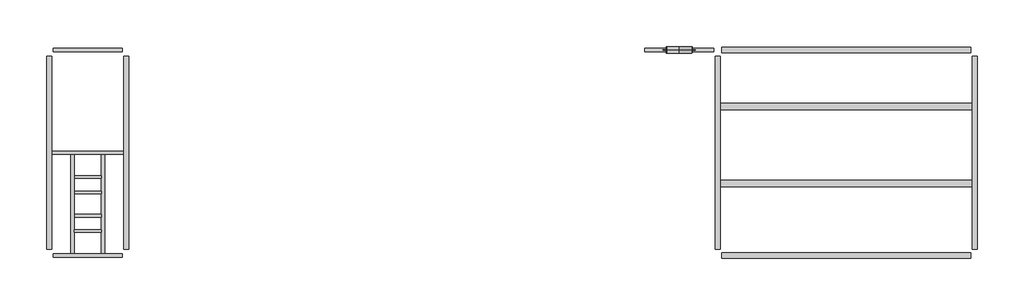
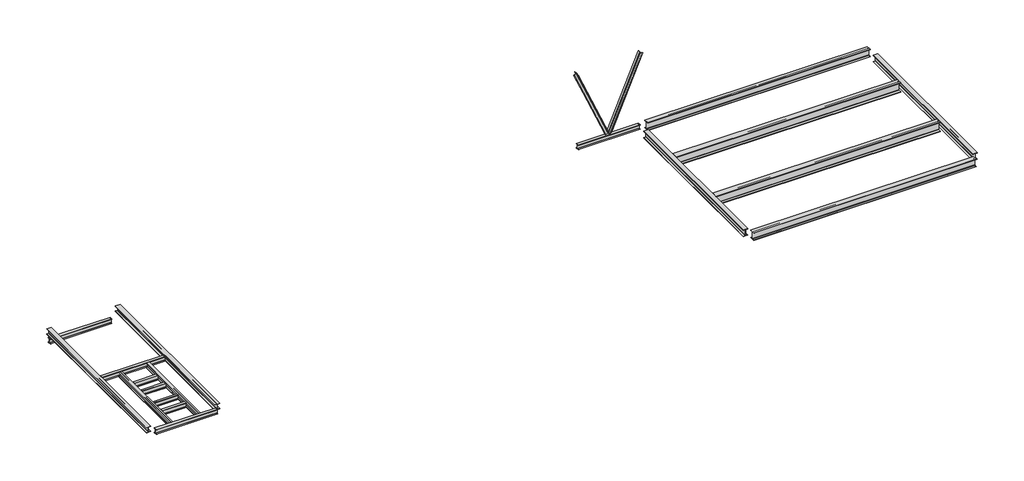
# One storey: 18 beams, 2 members.
"""IFC4 building model written with IfcOpenShell, lengths in millimetres."""

import ifcopenshell
import ifcopenshell.guid

model = None  # the IFC model being written
_history = None  # IfcOwnerHistory: only IFC2X3 demands one
_inside = {}  # id of a spatial element -> (the spatial element, [elements in it])
_under = {}  # id of a project, library or spatial element -> (it, [spatial elements below it])
_declared = {}  # id of a project -> (the project, [libraries it declares])
_typed = {}  # id of a type object -> (the type object, [elements of that type])
_made_of = {}  # id of a material, layer set ... -> (it, [elements and type objects made of it])


def new_model(schema):
    """Start an empty IFC model of exactly this schema.

    Asked for "IFC4X3", IfcOpenShell would pick the latest addendum, in which some entities
    have other attributes; the version numbers below select the first issue.
    IFC2X3 requires an IfcOwnerHistory on every rooted entity: one is made here for all.
    """
    global model, _history
    if schema == "IFC4X3":
        model = ifcopenshell.file(schema_version=(4, 3, 0, 0))
    else:
        model = ifcopenshell.file(schema=schema)
    _inside.clear()
    _under.clear()
    _declared.clear()
    _typed.clear()
    _made_of.clear()
    _history = None
    if model.schema == "IFC2X3":
        org = make("IfcOrganization", Name="unknown")
        user = make(
            "IfcPersonAndOrganization",
            ThePerson=make("IfcPerson", FamilyName="unknown"),
            TheOrganization=org,
        )
        app = make(
            "IfcApplication",
            ApplicationDeveloper=org,
            Version="unknown",
            ApplicationFullName="unknown",
            ApplicationIdentifier="unknown",
        )
        _history = make(
            "IfcOwnerHistory",
            OwningUser=user,
            OwningApplication=app,
            ChangeAction="ADDED",
            CreationDate=0,
        )
    return model


def make(cls, **values):
    """One entity of the class cls with the attributes given. An attribute that is None is left unset."""
    return model.create_entity(
        cls, **{name: value for name, value in values.items() if value is not None}
    )


def rooted(cls, **values):
    """An entity with a GlobalId (a new one), such as an element, a storey or a relation."""
    return make(cls, GlobalId=ifcopenshell.guid.new(), OwnerHistory=_history, **values)


def si_unit(unit_type, name, prefix=None):
    """IfcSIUnit, for example si_unit("LENGTHUNIT", "METRE", prefix="MILLI")."""
    return make("IfcSIUnit", UnitType=unit_type, Prefix=prefix, Name=name)


def assignment(units):
    """IfcUnitAssignment: the units of a project."""
    return None if units is None else make("IfcUnitAssignment", Units=units)


def point(xyz):
    """IfcCartesianPoint."""
    return None if xyz is None else make("IfcCartesianPoint", Coordinates=xyz)


def direction(xyz):
    """IfcDirection."""
    return None if xyz is None else make("IfcDirection", DirectionRatios=xyz)


def frame(location, z_axis=None, x_axis=None):
    """IfcAxis2Placement3D, a coordinate frame: its origin and axes. An axis left out is left unset."""
    return make(
        "IfcAxis2Placement3D",
        Location=point(location),
        Axis=direction(z_axis),
        RefDirection=direction(x_axis),
    )


def frame_2d(location, x_axis=None):
    """IfcAxis2Placement2D, a coordinate frame in the plane: its origin and x axis."""
    return make(
        "IfcAxis2Placement2D", Location=point(location), RefDirection=direction(x_axis)
    )


def origin():
    """The frame at (0, 0, 0) with its axes left unset."""
    return frame((0.0, 0.0, 0.0))


def place(relative_to, where):
    """IfcLocalPlacement: puts the frame where relative to a parent placement (None: the world)."""
    return make(
        "IfcLocalPlacement", PlacementRelTo=relative_to, RelativePlacement=where
    )


def context(
    kind, dimensions, precision=None, world=None, true_north=None, identifier=None
):
    """IfcGeometricRepresentationContext, for example the 3D "Model" context."""
    return make(
        "IfcGeometricRepresentationContext",
        ContextIdentifier=identifier,
        ContextType=kind,
        CoordinateSpaceDimension=dimensions,
        Precision=precision,
        WorldCoordinateSystem=world,
        TrueNorth=true_north,
    )


def project(units=None, contexts=None):
    """IfcProject with its units and contexts."""
    return rooted(
        "IfcProject",
        Name="project",
        RepresentationContexts=contexts,
        UnitsInContext=assignment(units),
    )


def spatial(cls, under=None, at=None, **own):
    """A site, building, storey or space (cls), placed at a placement, below another one or the project."""
    s = rooted(cls, ObjectPlacement=at, **own)
    if under is not None:
        _under.setdefault(under.id(), (under, []))[1].append(s)
    return s


def polyline(points):
    """IfcPolyline through the points."""
    return make("IfcPolyline", Points=[point(p) for p in points])


def circle_curve(where, radius):
    """IfcCircle in the frame where."""
    return make("IfcCircle", Position=where, Radius=radius)


def trimmed(basis, trim1, trim2, sense, master):
    """IfcTrimmedCurve: the piece of a basis curve between two trims."""
    return make(
        "IfcTrimmedCurve",
        BasisCurve=basis,
        Trim1=trim1,
        Trim2=trim2,
        SenseAgreement=sense,
        MasterRepresentation=master,
    )


def segment(curve, same_sense, transition):
    """IfcCompositeCurveSegment."""
    return make(
        "IfcCompositeCurveSegment",
        Transition=transition,
        SameSense=same_sense,
        ParentCurve=curve,
    )


def composite_curve(segments, self_intersect=None):
    """IfcCompositeCurve: segments joined end to end."""
    return make("IfcCompositeCurve", Segments=segments, SelfIntersect=self_intersect)


def outline(outer, holes=None, kind="AREA"):
    """IfcArbitraryClosedProfileDef: a profile drawn as a closed curve; with holes, ...WithVoids."""
    if holes is None:
        return make("IfcArbitraryClosedProfileDef", ProfileType=kind, OuterCurve=outer)
    return make(
        "IfcArbitraryProfileDefWithVoids",
        ProfileType=kind,
        OuterCurve=outer,
        InnerCurves=holes,
    )


def extrude(swept, where, along, depth):
    """IfcExtrudedAreaSolid: the profile swept, set in the frame where, extruded along a direction by depth."""
    return make(
        "IfcExtrudedAreaSolid",
        SweptArea=swept,
        Position=where,
        ExtrudedDirection=direction(along),
        Depth=depth,
    )


def shape(context_of_items, identifier, shape_type, items):
    """IfcShapeRepresentation: the items that make up one representation, for example the "Body"."""
    return make(
        "IfcShapeRepresentation",
        ContextOfItems=context_of_items,
        RepresentationIdentifier=identifier,
        RepresentationType=shape_type,
        Items=items,
    )


def source(mapping_origin, context_of_items, identifier, shape_type, items):
    """IfcRepresentationMap: a shape defined once, which mapped items show again and again."""
    return make(
        "IfcRepresentationMap",
        MappingOrigin=mapping_origin,
        MappedRepresentation=shape(context_of_items, identifier, shape_type, items),
    )


def transform(
    local_origin,
    x_axis=None,
    y_axis=None,
    z_axis=None,
    scale=None,
    scale2=None,
    scale3=None,
    uniform=True,
):
    """IfcCartesianTransformationOperator3D, or its non-uniform kind. x_axis, y_axis, z_axis: its Axis1, 2, 3."""
    if uniform:
        return make(
            "IfcCartesianTransformationOperator3D",
            Axis1=direction(x_axis),
            Axis2=direction(y_axis),
            LocalOrigin=point(local_origin),
            Scale=scale,
            Axis3=direction(z_axis),
        )
    return make(
        "IfcCartesianTransformationOperator3DnonUniform",
        Axis1=direction(x_axis),
        Axis2=direction(y_axis),
        LocalOrigin=point(local_origin),
        Scale=scale,
        Axis3=direction(z_axis),
        Scale2=scale2,
        Scale3=scale3,
    )


def mapped(mapping_source, mapping_target):
    """IfcMappedItem: shows the shape of a source again, moved by a transform."""
    return make(
        "IfcMappedItem", MappingSource=mapping_source, MappingTarget=mapping_target
    )


def made_of(thing, what):
    """Note that an element or type object is made of a material, layer set ...; save() writes the relation."""
    if what is not None:
        _made_of.setdefault(what.id(), (what, []))[1].append(thing)
    return thing


def element(
    cls,
    number,
    at=None,
    inside=None,
    cuts=None,
    type_object=None,
    material=None,
    context=None,
    identifier="Body",
    shape_type=None,
    held_by="IfcProductDefinitionShape",
    body=None,
    shapes=None,
    **own,
):
    """One element of the class cls, such as IfcWall. Its Tag is "e" and its number.

    at: its placement. inside: the storey or other place that contains it. cuts: it is an
    opening in that element (IfcRelVoidsElement). A single representation is given by context,
    identifier, shape_type and body (its items); several are given by shapes. held_by: the class
    of the entity that holds the representations. save() writes the other relations.
    """
    e = rooted(cls, Tag="e%d" % number, ObjectPlacement=at, **own)
    if body is not None:
        shapes = [shape(context, identifier, shape_type, body)]
    if shapes is not None:
        e.Representation = make(held_by, Representations=shapes)
    if inside is not None:
        _inside.setdefault(inside.id(), (inside, []))[1].append(e)
    if cuts is not None:
        rooted(
            "IfcRelVoidsElement", RelatingBuildingElement=cuts, RelatedOpeningElement=e
        )
    if type_object is not None:
        _typed.setdefault(type_object.id(), (type_object, []))[1].append(e)
    return made_of(e, material)


def aggregate(whole, parts):
    """IfcRelAggregates: a whole, such as a stair, and the parts it consists of."""
    return rooted("IfcRelAggregates", RelatingObject=whole, RelatedObjects=parts)


def save(model, path):
    """Write the relations noted so far, then the file.

    IfcRelAggregates (storeys below a building ...), IfcRelContainedInSpatialStructure (elements
    in a storey), IfcRelDefinesByType, IfcRelAssociatesMaterial and IfcRelDeclares: one each for
    every whole, place, type object, material and project.
    """
    for whole, parts in _under.values():
        aggregate(whole, parts)
    for where, things in _inside.values():
        rooted(
            "IfcRelContainedInSpatialStructure",
            RelatedElements=things,
            RelatingStructure=where,
        )
    for kind, things in _typed.values():
        rooted("IfcRelDefinesByType", RelatedObjects=things, RelatingType=kind)
    for what, things in _made_of.values():
        rooted("IfcRelAssociatesMaterial", RelatedObjects=things, RelatingMaterial=what)
    for by, libraries in _declared.values():
        rooted("IfcRelDeclares", RelatingContext=by, RelatedDefinitions=libraries)
    model.write(path)


def steel_framing_w_astm_a6m_f33feb28(model_context):
    return source(origin(), model_context, "Body", "SweptSolid", [
        extrude(outline(composite_curve([segment(polyline([(67.0, -94.8), (67.0, -105.0), (-67.0, -105.0), (-67.0, -94.8), (-10.775, -94.8)]), True, "CONTINUOUS"), segment(trimmed(circle_curve(frame_2d((-10.775, -87.2)), 7.6), [point((-10.775, -94.8))], [point((-3.175, -87.2))], True, "CARTESIAN"), True, "CONTINUOUS"), segment(polyline([(-3.175, -87.2), (-3.175, 87.2)]), True, "CONTINUOUS"), segment(trimmed(circle_curve(frame_2d((-10.775, 87.2)), 7.6), [point((-3.175, 87.2))], [point((-10.775, 94.8))], True, "CARTESIAN"), True, "CONTINUOUS"), segment(polyline([(-10.775, 94.8), (-67.0, 94.8), (-67.0, 105.0), (67.0, 105.0), (67.0, 94.8), (10.775, 94.8)]), True, "CONTINUOUS"), segment(trimmed(circle_curve(frame_2d((10.775, 87.2)), 7.6), [point((10.775, 94.8))], [point((3.175, 87.2))], True, "CARTESIAN"), True, "CONTINUOUS"), segment(polyline([(3.175, 87.2), (3.175, -87.2)]), True, "CONTINUOUS"), segment(trimmed(circle_curve(frame_2d((10.775, -87.2)), 7.6), [point((3.175, -87.2))], [point((10.775, -94.8))], True, "CARTESIAN"), True, "CONTINUOUS"), segment(polyline([(10.775, -94.8), (67.0, -94.8)]), True, "CONTINUOUS")], self_intersect=False)), frame((-1346.3, 0.0, 0.0), z_axis=(1.0, 0.0, 0.0), x_axis=(0.0, 1.0, 0.0)), (0.0, 0.0, 1.0), 2692.6),
    ])


def steel_framing_w_astm_a6m_fe1e75f4(model_context):
    return source(origin(), model_context, "Body", "SweptSolid", [
        extrude(outline(composite_curve([segment(polyline([(67.0, -94.8), (67.0, -105.0), (-67.0, -105.0), (-67.0, -94.8), (-10.775, -94.8)]), True, "CONTINUOUS"), segment(trimmed(circle_curve(frame_2d((-10.775, -87.2)), 7.6), [point((-10.775, -94.8))], [point((-3.175, -87.2))], True, "CARTESIAN"), True, "CONTINUOUS"), segment(polyline([(-3.175, -87.2), (-3.175, 87.2)]), True, "CONTINUOUS"), segment(trimmed(circle_curve(frame_2d((-10.775, 87.2)), 7.6), [point((-3.175, 87.2))], [point((-10.775, 94.8))], True, "CARTESIAN"), True, "CONTINUOUS"), segment(polyline([(-10.775, 94.8), (-67.0, 94.8), (-67.0, 105.0), (67.0, 105.0), (67.0, 94.8), (10.775, 94.8)]), True, "CONTINUOUS"), segment(trimmed(circle_curve(frame_2d((10.775, 87.2)), 7.6), [point((10.775, 94.8))], [point((3.175, 87.2))], True, "CARTESIAN"), True, "CONTINUOUS"), segment(polyline([(3.175, 87.2), (3.175, -87.2)]), True, "CONTINUOUS"), segment(trimmed(circle_curve(frame_2d((10.775, -87.2)), 7.6), [point((3.175, -87.2))], [point((10.775, -94.8))], True, "CARTESIAN"), True, "CONTINUOUS"), segment(polyline([(10.775, -94.8), (67.0, -94.8)]), True, "CONTINUOUS")], self_intersect=False)), frame((-1386.3, 0.0, 0.0), z_axis=(1.0, 0.0, 0.0), x_axis=(0.0, 1.0, 0.0)), (0.0, 0.0, 1.0), 2772.6),
    ])


def steel_framing_w_astm_a6m_8cea9429(model_context):
    return source(origin(), model_context, "Body", "SweptSolid", [
        extrude(outline(composite_curve([segment(polyline([(101.5, -137.9), (101.5, -151.0), (-101.5, -151.0), (-101.5, -137.9), (-16.545, -137.9)]), True, "CONTINUOUS"), segment(trimmed(circle_curve(frame_2d((-16.545, -125.1)), 12.8), [point((-16.545, -137.9))], [point((-3.745, -125.1))], True, "CARTESIAN"), True, "CONTINUOUS"), segment(polyline([(-3.745, -125.1), (-3.745, 125.1)]), True, "CONTINUOUS"), segment(trimmed(circle_curve(frame_2d((-16.545, 125.1)), 12.8), [point((-3.745, 125.1))], [point((-16.545, 137.9))], True, "CARTESIAN"), True, "CONTINUOUS"), segment(polyline([(-16.545, 137.9), (-101.5, 137.9), (-101.5, 151.0), (101.5, 151.0), (101.5, 137.9), (16.545, 137.9)]), True, "CONTINUOUS"), segment(trimmed(circle_curve(frame_2d((16.545, 125.1)), 12.8), [point((16.545, 137.9))], [point((3.745, 125.1))], True, "CARTESIAN"), True, "CONTINUOUS"), segment(polyline([(3.745, 125.1), (3.745, -125.1)]), True, "CONTINUOUS"), segment(trimmed(circle_curve(frame_2d((16.545, -125.1)), 12.8), [point((3.745, -125.1))], [point((16.545, -137.9))], True, "CARTESIAN"), True, "CONTINUOUS"), segment(polyline([(16.545, -137.9), (101.5, -137.9)]), True, "CONTINUOUS")], self_intersect=False)), frame((-3753.8, 0.0, 0.0), z_axis=(1.0, 0.0, 0.0), x_axis=(0.0, 1.0, 0.0)), (0.0, 0.0, 1.0), 7507.6),
    ])


def steel_framing_w_astm_a6m_fd2852ff(model_context):
    return source(origin(), model_context, "Body", "SweptSolid", [
        extrude(outline(composite_curve([segment(polyline([(67.0, -94.8), (67.0, -105.0), (-67.0, -105.0), (-67.0, -94.8), (-10.775, -94.8)]), True, "CONTINUOUS"), segment(trimmed(circle_curve(frame_2d((-10.775, -87.2)), 7.6), [point((-10.775, -94.8))], [point((-3.175, -87.2))], True, "CARTESIAN"), True, "CONTINUOUS"), segment(polyline([(-3.175, -87.2), (-3.175, 87.2)]), True, "CONTINUOUS"), segment(trimmed(circle_curve(frame_2d((-10.775, 87.2)), 7.6), [point((-3.175, 87.2))], [point((-10.775, 94.8))], True, "CARTESIAN"), True, "CONTINUOUS"), segment(polyline([(-10.775, 94.8), (-67.0, 94.8), (-67.0, 105.0), (67.0, 105.0), (67.0, 94.8), (10.775, 94.8)]), True, "CONTINUOUS"), segment(trimmed(circle_curve(frame_2d((10.775, 87.2)), 7.6), [point((10.775, 94.8))], [point((3.175, 87.2))], True, "CARTESIAN"), True, "CONTINUOUS"), segment(polyline([(3.175, 87.2), (3.175, -87.2)]), True, "CONTINUOUS"), segment(trimmed(circle_curve(frame_2d((10.775, -87.2)), 7.6), [point((3.175, -87.2))], [point((10.775, -94.8))], True, "CARTESIAN"), True, "CONTINUOUS"), segment(polyline([(10.775, -94.8), (67.0, -94.8)]), True, "CONTINUOUS")], self_intersect=False)), frame((-1920.3, 0.0, 0.0), z_axis=(1.0, 0.0, 0.0), x_axis=(0.0, 1.0, 0.0)), (0.0, 0.0, 1.0), 3840.6),
    ])


def steel_framing_w_astm_a6m_80da07c9(model_context):
    return source(origin(), model_context, "Body", "SweptSolid", [
        extrude(outline(composite_curve([segment(polyline([(101.0, -112.5), (101.0, -123.5), (-101.0, -123.5), (-101.0, -112.5), (-16.385, -112.5)]), True, "CONTINUOUS"), segment(trimmed(circle_curve(frame_2d((-16.385, -99.8)), 12.7), [point((-16.385, -112.5))], [point((-3.685, -99.8))], True, "CARTESIAN"), True, "CONTINUOUS"), segment(polyline([(-3.685, -99.8), (-3.685, 99.8)]), True, "CONTINUOUS"), segment(trimmed(circle_curve(frame_2d((-16.385, 99.8)), 12.7), [point((-3.685, 99.8))], [point((-16.385, 112.5))], True, "CARTESIAN"), True, "CONTINUOUS"), segment(polyline([(-16.385, 112.5), (-101.0, 112.5), (-101.0, 123.5), (101.0, 123.5), (101.0, 112.5), (16.385, 112.5)]), True, "CONTINUOUS"), segment(trimmed(circle_curve(frame_2d((16.385, 99.8)), 12.7), [point((16.385, 112.5))], [point((3.685, 99.8))], True, "CARTESIAN"), True, "CONTINUOUS"), segment(polyline([(3.685, 99.8), (3.685, -99.8)]), True, "CONTINUOUS"), segment(trimmed(circle_curve(frame_2d((16.385, -99.8)), 12.7), [point((3.685, -99.8))], [point((16.385, -112.5))], True, "CARTESIAN"), True, "CONTINUOUS"), segment(polyline([(16.385, -112.5), (101.0, -112.5)]), True, "CONTINUOUS")], self_intersect=False)), frame((-3753.8, 0.0, 0.0), z_axis=(1.0, 0.0, 0.0), x_axis=(0.0, 1.0, 0.0)), (0.0, 0.0, 1.0), 7507.6),
    ])


def steel_framing_w_astm_a6m_f88b2983(model_context):
    return source(origin(), model_context, "Body", "SweptSolid", [
        extrude(outline(composite_curve([segment(polyline([(51.0, -95.0), (51.0, -103.0), (-51.0, -103.0), (-51.0, -95.0), (-10.71, -95.0)]), True, "CONTINUOUS"), segment(trimmed(circle_curve(frame_2d((-10.71, -87.4)), 7.6), [point((-10.71, -95.0))], [point((-3.11, -87.4))], True, "CARTESIAN"), True, "CONTINUOUS"), segment(polyline([(-3.11, -87.4), (-3.11, 87.4)]), True, "CONTINUOUS"), segment(trimmed(circle_curve(frame_2d((-10.71, 87.4)), 7.6), [point((-3.11, 87.4))], [point((-10.71, 95.0))], True, "CARTESIAN"), True, "CONTINUOUS"), segment(polyline([(-10.71, 95.0), (-51.0, 95.0), (-51.0, 103.0), (51.0, 103.0), (51.0, 95.0), (10.71, 95.0)]), True, "CONTINUOUS"), segment(trimmed(circle_curve(frame_2d((10.71, 87.4)), 7.6), [point((10.71, 95.0))], [point((3.11, 87.4))], True, "CARTESIAN"), True, "CONTINUOUS"), segment(polyline([(3.11, 87.4), (3.11, -87.4)]), True, "CONTINUOUS"), segment(trimmed(circle_curve(frame_2d((10.71, -87.4)), 7.6), [point((3.11, -87.4))], [point((10.71, -95.0))], True, "CARTESIAN"), True, "CONTINUOUS"), segment(polyline([(10.71, -95.0), (51.0, -95.0)]), True, "CONTINUOUS")], self_intersect=False)), frame((-520.3, 0.0, 0.0), z_axis=(1.0, 0.0, 0.0), x_axis=(0.0, 1.0, 0.0)), (0.0, 0.0, 1.0), 1040.6),
    ])


def steel_framing_w_astm_a6m_d888c6d0(model_context):
    return source(origin(), model_context, "Body", "SweptSolid", [
        extrude(outline(composite_curve([segment(polyline([(102.5, -159.7), (102.5, -176.5), (-102.5, -176.5), (-102.5, -159.7), (-19.7, -159.7)]), True, "CONTINUOUS"), segment(trimmed(circle_curve(frame_2d((-19.7, -144.7)), 15.0), [point((-19.7, -159.7))], [point((-4.7, -144.7))], True, "CARTESIAN"), True, "CONTINUOUS"), segment(polyline([(-4.7, -144.7), (-4.7, 144.7)]), True, "CONTINUOUS"), segment(trimmed(circle_curve(frame_2d((-19.7, 144.7)), 15.0), [point((-4.7, 144.7))], [point((-19.7, 159.7))], True, "CARTESIAN"), True, "CONTINUOUS"), segment(polyline([(-19.7, 159.7), (-102.5, 159.7), (-102.5, 176.5), (102.5, 176.5), (102.5, 159.7), (19.7, 159.7)]), True, "CONTINUOUS"), segment(trimmed(circle_curve(frame_2d((19.7, 144.7)), 15.0), [point((19.7, 159.7))], [point((4.7, 144.7))], True, "CARTESIAN"), True, "CONTINUOUS"), segment(polyline([(4.7, 144.7), (4.7, -144.7)]), True, "CONTINUOUS"), segment(trimmed(circle_curve(frame_2d((19.7, -144.7)), 15.0), [point((4.7, -144.7))], [point((19.7, -159.7))], True, "CARTESIAN"), True, "CONTINUOUS"), segment(polyline([(19.7, -159.7), (102.5, -159.7)]), True, "CONTINUOUS")], self_intersect=False)), frame((-4846.3, 0.0, 0.0), z_axis=(1.0, 0.0, 0.0), x_axis=(0.0, 1.0, 0.0)), (0.0, 0.0, 1.0), 9692.6),
    ])


def steel_framing_w_astm_a6m_4c16a149(model_context):
    return source(origin(), model_context, "Body", "SweptSolid", [
        extrude(outline(composite_curve([segment(polyline([(131.0, -190.2), (131.0, -209.5), (-131.0, -209.5), (-131.0, -190.2), (-16.0, -190.2)]), True, "CONTINUOUS"), segment(trimmed(circle_curve(frame_2d((-16.0, -180.0)), 10.2), [point((-16.0, -190.2))], [point((-5.8, -180.0))], True, "CARTESIAN"), True, "CONTINUOUS"), segment(polyline([(-5.8, -180.0), (-5.8, 180.0)]), True, "CONTINUOUS"), segment(trimmed(circle_curve(frame_2d((-16.0, 180.0)), 10.2), [point((-5.8, 180.0))], [point((-16.0, 190.2))], True, "CARTESIAN"), True, "CONTINUOUS"), segment(polyline([(-16.0, 190.2), (-131.0, 190.2), (-131.0, 209.5), (131.0, 209.5), (131.0, 190.2), (16.0, 190.2)]), True, "CONTINUOUS"), segment(trimmed(circle_curve(frame_2d((16.0, 180.0)), 10.2), [point((16.0, 190.2))], [point((5.8, 180.0))], True, "CARTESIAN"), True, "CONTINUOUS"), segment(polyline([(5.8, 180.0), (5.8, -180.0)]), True, "CONTINUOUS"), segment(trimmed(circle_curve(frame_2d((16.0, -180.0)), 10.2), [point((5.8, -180.0))], [point((16.0, -190.2))], True, "CARTESIAN"), True, "CONTINUOUS"), segment(polyline([(16.0, -190.2), (131.0, -190.2)]), True, "CONTINUOUS")], self_intersect=False)), frame((-4885.8, 0.0, 0.0), z_axis=(1.0, 0.0, 0.0), x_axis=(0.0, 1.0, 0.0)), (0.0, 0.0, 1.0), 9771.6),
    ])


def member_96e87236(model_context):
    return source(origin(), model_context, "Body", "SweptSolid", [
        extrude(outline(composite_curve([segment(polyline([(0.0, 36.4), (130.0, 36.4)]), True, "CONTINUOUS"), segment(trimmed(circle_curve(frame_2d((118.0, 36.4)), 12.0), [point((130.0, 36.4))], [point((118.0, 24.4))], False, "CARTESIAN"), True, "CONTINUOUS"), segment(polyline([(118.0, 24.4), (24.0, 24.4)]), True, "CONTINUOUS"), segment(trimmed(circle_curve(frame_2d((24.0, 12.4)), 12.0), [point((24.0, 24.4))], [point((12.0, 12.4))], True, "CARTESIAN"), True, "CONTINUOUS"), segment(polyline([(12.0, 12.4), (12.0, -81.6)]), True, "CONTINUOUS"), segment(trimmed(circle_curve(frame_2d((0.0, -81.6)), 12.0), [point((12.0, -81.6))], [point((0.0, -93.6))], False, "CARTESIAN"), True, "CONTINUOUS"), segment(polyline([(0.0, -93.6), (0.0, 36.4)]), True, "CONTINUOUS")], self_intersect=False)), frame((-1749.149537, 0.0, 0.0), z_axis=(1.0, 0.0, 0.0), x_axis=(0.0, 1.0, 0.0)), (0.0, 0.0, 1.0), 3498.299074),
        extrude(outline(composite_curve([segment(polyline([(0.0, 36.4), (0.0, -93.6)]), True, "CONTINUOUS"), segment(trimmed(circle_curve(frame_2d((0.0, -81.6)), 12.0), [point((0.0, -93.6))], [point((-12.0, -81.6))], False, "CARTESIAN"), True, "CONTINUOUS"), segment(polyline([(-12.0, -81.6), (-12.0, 12.4)]), True, "CONTINUOUS"), segment(trimmed(circle_curve(frame_2d((-24.0, 12.4)), 12.0), [point((-12.0, 12.4))], [point((-24.0, 24.4))], True, "CARTESIAN"), True, "CONTINUOUS"), segment(polyline([(-24.0, 24.4), (-118.0, 24.4)]), True, "CONTINUOUS"), segment(trimmed(circle_curve(frame_2d((-118.0, 36.4)), 12.0), [point((-118.0, 24.4))], [point((-130.0, 36.4))], False, "CARTESIAN"), True, "CONTINUOUS"), segment(polyline([(-130.0, 36.4), (0.0, 36.4)]), True, "CONTINUOUS")], self_intersect=False)), frame((-1749.149537, 0.0, 0.0), z_axis=(1.0, 0.0, 0.0), x_axis=(0.0, 1.0, 0.0)), (0.0, 0.0, 1.0), 3498.299074),
    ])


model = new_model("IFC4")

# Units and contexts
model_context = context("Model", 3, world=origin())
ifc_project = project(units=[si_unit("LENGTHUNIT", "METRE", prefix="MILLI")], contexts=[model_context])

# Site, building, storey
site = spatial("IfcSite", under=ifc_project)
building = spatial("IfcBuilding", under=site)
storey = spatial("IfcBuildingStorey", under=building, Name="T.O.S(4)", Elevation=5219.8243501)

# Beams
placement = place(None, origin())
steel_framing_w_astm_a6m_shape = steel_framing_w_astm_a6m_f33feb28(model_context)
element("IfcBeam", 1, ObjectType="Steel Framing_W_ASTM A6M : H_SB_AR_S02_W200x31.3_B6", at=placement, inside=storey, context=model_context, shape_type="MappedRepresentation", body=[
    mapped(steel_framing_w_astm_a6m_shape, transform((1500.0, 22499.5208589, 4214.8243501), x_axis=(1.0, 0.0, 0.0), y_axis=(0.0, 1.0, 0.0), z_axis=(0.0, 0.0, 1.0))),
])
element("IfcBeam", 2, ObjectType="Steel Framing_W_ASTM A6M : H_SB_AR_S02_W200x31.3_B6", at=placement, inside=storey, context=model_context, shape_type="MappedRepresentation", body=[
    mapped(steel_framing_w_astm_a6m_shape, transform((1500.0, 14499.5208589, 4899.8243501), x_axis=(1.0, 0.0, 0.0), y_axis=(0.0, 1.0, 0.0), z_axis=(0.0, 0.0, 1.0))),
])
element("IfcBeam", 3, ObjectType="Steel Framing_W_ASTM A6M : H_SB_AR_S02_W200x31.3_B6", at=placement, inside=storey, context=model_context, shape_type="MappedRepresentation", body=[
    mapped(steel_framing_w_astm_a6m_shape, transform((24500.0, 22499.5208589, 5114.8243501), x_axis=(1.0, 0.0, 0.0), y_axis=(0.0, 1.0, 0.0), z_axis=(0.0, 0.0, 1.0))),
])
steel_framing_w_astm_a6m_2_shape = steel_framing_w_astm_a6m_fe1e75f4(model_context)
element("IfcBeam", 4, ObjectType="Steel Framing_W_ASTM A6M : H_SB_AR_S02_W200x31.3_B6", at=placement, inside=storey, context=model_context, shape_type="MappedRepresentation", body=[
    mapped(steel_framing_w_astm_a6m_2_shape, transform((1500.0, 18499.5208589, 4899.8243501), x_axis=(1.0, 0.0, 0.0), y_axis=(0.0, 1.0, 0.0), z_axis=(0.0, 0.0, 1.0))),
])
steel_framing_w_astm_a6m_3_shape = steel_framing_w_astm_a6m_8cea9429(model_context)
element("IfcBeam", 5, ObjectType="Steel Framing_W_ASTM A6M : H_SB_AR_S02_W310x60_G4", at=placement, inside=storey, context=model_context, shape_type="MappedRepresentation", body=[
    mapped(steel_framing_w_astm_a6m_3_shape, transform((26000.0, 18499.5208589, 4853.8243501), x_axis=(0.0, 1.0, 0.0), y_axis=(-1.0, 0.0, 0.0), z_axis=(0.0, 0.0, 1.0))),
])
element("IfcBeam", 6, ObjectType="Steel Framing_W_ASTM A6M : H_SB_AR_S02_W310x60_G4", at=placement, inside=storey, context=model_context, shape_type="MappedRepresentation", body=[
    mapped(steel_framing_w_astm_a6m_3_shape, transform((36000.0, 18499.5208589, 4853.8243501), x_axis=(0.0, 1.0, 0.0), y_axis=(-1.0, 0.0, 0.0), z_axis=(0.0, 0.0, 1.0))),
])
steel_framing_w_astm_a6m_4_shape = steel_framing_w_astm_a6m_fd2852ff(model_context)
element("IfcBeam", 7, ObjectType="Steel Framing_W_ASTM A6M : H_SB_AR_S02_W200x31.3_B6", at=placement, inside=storey, context=model_context, shape_type="MappedRepresentation", body=[
    mapped(steel_framing_w_astm_a6m_4_shape, transform((900.0, 16499.5208589, 4899.8243501), x_axis=(0.0, -1.0, 0.0), y_axis=(1.0, 0.0, 0.0), z_axis=(0.0, 0.0, 1.0))),
])
element("IfcBeam", 8, ObjectType="Steel Framing_W_ASTM A6M : H_SB_AR_S02_W200x31.3_B6", at=placement, inside=storey, context=model_context, shape_type="MappedRepresentation", body=[
    mapped(steel_framing_w_astm_a6m_4_shape, transform((2100.0, 16499.5208589, 4899.8243501), x_axis=(0.0, -1.0, 0.0), y_axis=(1.0, 0.0, 0.0), z_axis=(0.0, 0.0, 1.0))),
])
steel_framing_w_astm_a6m_5_shape = steel_framing_w_astm_a6m_80da07c9(model_context)
element("IfcBeam", 9, ObjectType="Steel Framing_W_ASTM A6M : H_SB_AR_S02_W250x49.1_G5", at=placement, inside=storey, context=model_context, shape_type="MappedRepresentation", body=[
    mapped(steel_framing_w_astm_a6m_5_shape, transform((0.0, 18499.5208589, 4881.3243501), x_axis=(0.0, 1.0, 0.0), y_axis=(-1.0, 0.0, 0.0), z_axis=(0.0, 0.0, 1.0))),
])
element("IfcBeam", 10, ObjectType="Steel Framing_W_ASTM A6M : H_SB_AR_S02_W250x49.1_G5", at=placement, inside=storey, context=model_context, shape_type="MappedRepresentation", body=[
    mapped(steel_framing_w_astm_a6m_5_shape, transform((3000.0, 18499.5208589, 4881.3243501), x_axis=(0.0, -1.0, 0.0), y_axis=(1.0, 0.0, 0.0), z_axis=(0.0, 0.0, 1.0))),
])
steel_framing_w_astm_a6m_6_shape = steel_framing_w_astm_a6m_f88b2983(model_context)
element("IfcBeam", 11, ObjectType="Steel Framing_W_ASTM A6M : H_SB_AR_S02_W200x22.5_J1", at=placement, inside=storey, context=model_context, shape_type="MappedRepresentation", body=[
    mapped(steel_framing_w_astm_a6m_6_shape, transform((1500.0, 17549.5208589, 4901.8243501), x_axis=(1.0, 0.0, 0.0), y_axis=(0.0, 1.0, 0.0), z_axis=(0.0, 0.0, 1.0))),
])
element("IfcBeam", 12, ObjectType="Steel Framing_W_ASTM A6M : H_SB_AR_S02_W200x22.5_J1", at=placement, inside=storey, context=model_context, shape_type="MappedRepresentation", body=[
    mapped(steel_framing_w_astm_a6m_6_shape, transform((1500.0, 16949.5208589, 4901.8243501), x_axis=(1.0, 0.0, 0.0), y_axis=(0.0, 1.0, 0.0), z_axis=(0.0, 0.0, 1.0))),
])
element("IfcBeam", 13, ObjectType="Steel Framing_W_ASTM A6M : H_SB_AR_S02_W200x22.5_J1", at=placement, inside=storey, context=model_context, shape_type="MappedRepresentation", body=[
    mapped(steel_framing_w_astm_a6m_6_shape, transform((1500.0, 16049.5208589, 4901.8243501), x_axis=(1.0, 0.0, 0.0), y_axis=(0.0, 1.0, 0.0), z_axis=(0.0, 0.0, 1.0))),
])
element("IfcBeam", 14, ObjectType="Steel Framing_W_ASTM A6M : H_SB_AR_S02_W200x22.5_J1", at=placement, inside=storey, context=model_context, shape_type="MappedRepresentation", body=[
    mapped(steel_framing_w_astm_a6m_6_shape, transform((1500.0, 15449.5208589, 4901.8243501), x_axis=(1.0, 0.0, 0.0), y_axis=(0.0, 1.0, 0.0), z_axis=(0.0, 0.0, 1.0))),
])
steel_framing_w_astm_a6m_7_shape = steel_framing_w_astm_a6m_d888c6d0(model_context)
element("IfcBeam", 15, ObjectType="Steel Framing_W_ASTM A6M : H_SB_AR_S02_W360x79_B2", at=placement, inside=storey, context=model_context, shape_type="MappedRepresentation", body=[
    mapped(steel_framing_w_astm_a6m_7_shape, transform((31000.0, 22499.5208589, 5043.3243501), x_axis=(1.0, 0.0, 0.0), y_axis=(0.0, 1.0, 0.0), z_axis=(0.0, 0.0, 1.0))),
])
element("IfcBeam", 16, ObjectType="Steel Framing_W_ASTM A6M : H_SB_AR_S02_W360x79_B2", at=placement, inside=storey, context=model_context, shape_type="MappedRepresentation", body=[
    mapped(steel_framing_w_astm_a6m_7_shape, transform((31000.0, 14499.5208589, 4828.3243501), x_axis=(1.0, 0.0, 0.0), y_axis=(0.0, 1.0, 0.0), z_axis=(0.0, 0.0, 1.0))),
])
steel_framing_w_astm_a6m_8_shape = steel_framing_w_astm_a6m_4c16a149(model_context)
element("IfcBeam", 17, ObjectType="Steel Framing_W_ASTM A6M : H_SB_AR_S02_W410x114_B9", at=placement, inside=storey, context=model_context, shape_type="MappedRepresentation", body=[
    mapped(steel_framing_w_astm_a6m_8_shape, transform((31000.0, 20299.5208589, 4795.3243501), x_axis=(1.0, 0.0, 0.0), y_axis=(0.0, 1.0, 0.0), z_axis=(0.0, 0.0, 1.0))),
])
element("IfcBeam", 18, ObjectType="Steel Framing_W_ASTM A6M : H_SB_AR_S02_W410x114_B9", at=placement, inside=storey, context=model_context, shape_type="MappedRepresentation", body=[
    mapped(steel_framing_w_astm_a6m_8_shape, transform((31000.0, 17299.5208589, 4795.3243501), x_axis=(1.0, 0.0, 0.0), y_axis=(0.0, 1.0, 0.0), z_axis=(0.0, 0.0, 1.0))),
])

# Members
member_shape = member_96e87236(model_context)
element("IfcMember", 19, ObjectType="0123_Steel Framing_2Ls-KSD3502 : H_SB_AR_S04_2Ls-130x130x12_VBR1", at=placement, inside=storey, context=model_context, shape_type="MappedRepresentation", body=[
    mapped(member_shape, transform((25223.7124521, 22499.5208589, 6876.090442), x_axis=(0.39391929857916597, 0.0, 0.9191450300180586), y_axis=(0.0, 1.0, 0.0), z_axis=(-0.9191450300180586, 0.0, 0.39391929857916597))),
])
element("IfcMember", 20, ObjectType="0123_Steel Framing_2Ls-KSD3502 : H_SB_AR_S04_2Ls-130x130x12_VBR1", at=placement, inside=storey, context=model_context, shape_type="MappedRepresentation", body=[
    mapped(member_shape, transform((23776.2875479, 22499.5208589, 6876.090442), x_axis=(0.3939192985791688, 0.0, -0.9191450300180575), y_axis=(0.0, 1.0, 0.0), z_axis=(0.9191450300180575, 0.0, 0.3939192985791688))),
])

save(model, "model.ifc")

# Revit data of these elements
# Type "Steel Framing_W_ASTM A6M : H_SB_AR_S02_W200x31.3_B6"
#   Type Mark = "B6"
#   Section Name Key = "W8x21"
#   Width = 13.4 cm
#   Web Thickness = 0.635 cm
#   Web Fillet = 0.76 cm
#   Warping Constant = 40800.0 cm⁶
#   Torsional Moment of Inertia = 11.70 cm⁴
#   Section Area = 39.7 cm²
#   Plastic Modulus weak axis = 93.2 cm³
#   Plastic Modulus strong axis = 334.0 cm³
#   Perimeter = 0.93 m²/m
#   Nominal Weight = 31.30 kgf/m
#   Moment of Inertia weak axis = 407.00 cm⁴
#   Moment of Inertia strong axis = 3130.00 cm⁴
#   Height = 21.0 cm
#   Flange Thickness = 1.02 cm
#   Elastic Modulus weak axis = 60.8 cm³
#   Elastic Modulus strong axis = 298.0 cm³
#   Centroid Vertical = 10.5 cm
#   Centroid Horizontal = 6.7 cm
#   Length [instance default] = 1500 mm
#   Structural Material [instance default] = Steel, 45-345
#   Bolt Spacing = 0
#   Assembly Code = ""
# Type "Steel Framing_W_ASTM A6M : H_SB_AR_S02_W310x60_G4"
#   Type Mark = "G4"
#   Section Name Key = "W12x40"
#   Width = 20.3 cm
#   Web Thickness = 0.749 cm
#   Web Fillet = 1.28 cm
#   Warping Constant = 387000.0 cm⁶
#   Torsional Moment of Inertia = 37.70 cm⁴
#   Section Area = 75.5 cm²
#   Plastic Modulus weak axis = 275.0 cm³
#   Plastic Modulus strong axis = 934.0 cm³
#   Perimeter = 1.38 m²/m
#   Nominal Weight = 60.00 kgf/m
#   Moment of Inertia weak axis = 1840.00 cm⁴
#   Moment of Inertia strong axis = 12800.00 cm⁴
#   Height = 30.2 cm
#   Flange Thickness = 1.31 cm
#   Elastic Modulus weak axis = 180.0 cm³
#   Elastic Modulus strong axis = 844.0 cm³
#   Centroid Vertical = 15.1 cm
#   Centroid Horizontal = 10.15 cm
#   Length [instance default] = 1500 mm
#   Structural Material [instance default] = Steel, 45-345
#   Bolt Spacing = 0
#   Assembly Code = ""
# Type "Steel Framing_W_ASTM A6M : H_SB_AR_S02_W250x49.1_G5"
#   Type Mark = "G5"
#   Section Name Key = "W10x33"
#   Width = 20.2 cm
#   Web Thickness = 0.737 cm
#   Web Fillet = 1.27 cm
#   Warping Constant = 212000.0 cm⁶
#   Torsional Moment of Inertia = 24.30 cm⁴
#   Section Area = 62.6 cm²
#   Plastic Modulus weak axis = 229.0 cm³
#   Plastic Modulus strong axis = 636.0 cm³
#   Perimeter = 1.27 m²/m
#   Nominal Weight = 49.10 kgf/m
#   Moment of Inertia weak axis = 1520.00 cm⁴
#   Moment of Inertia strong axis = 7120.00 cm⁴
#   Height = 24.7 cm
#   Flange Thickness = 1.1 cm
#   Elastic Modulus weak axis = 151.0 cm³
#   Elastic Modulus strong axis = 574.0 cm³
#   Centroid Vertical = 12.35 cm
#   Centroid Horizontal = 10.1 cm
#   Length [instance default] = 1500 mm
#   Structural Material [instance default] = Steel, 45-345
#   Bolt Spacing = 0
#   Assembly Code = ""
# Type "Steel Framing_W_ASTM A6M : H_SB_AR_S02_W200x22.5_J1"
#   Section Name Key = "W8x15"
#   Width = 10.2 cm
#   Web Thickness = 0.622 cm
#   Web Fillet = 0.76 cm
#   Warping Constant = 13900.0 cm⁶
#   Torsional Moment of Inertia = 5.70 cm⁴
#   Section Area = 28.6 cm²
#   Plastic Modulus weak axis = 43.8 cm³
#   Plastic Modulus strong axis = 223.0 cm³
#   Perimeter = 0.795 m²/m
#   Nominal Weight = 22.50 kgf/m
#   Moment of Inertia weak axis = 142.00 cm⁴
#   Moment of Inertia strong axis = 2000.00 cm⁴
#   Height = 20.6 cm
#   Flange Thickness = 0.8 cm
#   Elastic Modulus weak axis = 27.9 cm³
#   Elastic Modulus strong axis = 193.0 cm³
#   Centroid Vertical = 10.3 cm
#   Centroid Horizontal = 5.1 cm
#   Length [instance default] = 1500 mm
#   Structural Material [instance default] = Steel, 45-345
#   Bolt Spacing = 0
#   Assembly Code = ""
# Type "Steel Framing_W_ASTM A6M : H_SB_AR_S02_W360x79_B2"
#   Section Name Key = "W14x53"
#   Width = 20.5 cm
#   Web Thickness = 0.94 cm
#   Web Fillet = 1.5 cm
#   Warping Constant = 682000.0 cm⁶
#   Torsional Moment of Inertia = 80.70 cm⁴
#   Section Area = 101.0 cm²
#   Plastic Modulus weak axis = 361.0 cm³
#   Plastic Modulus strong axis = 1430.0 cm³
#   Perimeter = 1.48 m²/m
#   Nominal Weight = 79.00 kgf/m
#   Moment of Inertia weak axis = 2400.00 cm⁴
#   Moment of Inertia strong axis = 22500.00 cm⁴
#   Height = 35.3 cm
#   Flange Thickness = 1.68 cm
#   Elastic Modulus weak axis = 234.0 cm³
#   Elastic Modulus strong axis = 1270.0 cm³
#   Centroid Vertical = 17.65 cm
#   Centroid Horizontal = 10.25 cm
#   Length [instance default] = 1500 mm
#   Structural Material [instance default] = Steel, 45-345
#   Bolt Spacing = 0
#   Assembly Code = ""
# Type "Steel Framing_W_ASTM A6M : H_SB_AR_S02_W410x114_B9"
#   Section Name Key = "W16x77"
#   Width = 26.2 cm
#   Web Thickness = 1.16 cm
#   Web Fillet = 1.02 cm
#   Warping Constant = 2310000.0 cm⁶
#   Torsional Moment of Inertia = 149.00 cm⁴
#   Section Area = 146.0 cm²
#   Plastic Modulus weak axis = 674.0 cm³
#   Plastic Modulus strong axis = 2460.0 cm³
#   Perimeter = 1.84 m²/m
#   Nominal Weight = 114.00 kgf/m
#   Moment of Inertia weak axis = 5740.00 cm⁴
#   Moment of Inertia strong axis = 46200.00 cm⁴
#   Height = 41.9 cm
#   Flange Thickness = 1.93 cm
#   Elastic Modulus weak axis = 441.0 cm³
#   Elastic Modulus strong axis = 2200.0 cm³
#   Centroid Vertical = 20.95 cm
#   Centroid Horizontal = 13.1 cm
#   Length [instance default] = 1500 mm
#   Structural Material [instance default] = Steel, 45-345
#   Bolt Spacing = 0
#   Assembly Code = ""
# Type "0123_Steel Framing_2Ls-KSD3502 : H_SB_AR_S04_2Ls-130x130x12_VBR1"
#   Assembly Code = "B10"
#   Legs = "SLBB"
#   W = 8.97
#   Perimeter = 1.04 m²/m
#   Nominal Weight = 46.80 kgf/m
#   Length [instance default] = 1000 mm
#   Space = 0 mm
#   b = 130 mm
#   d = 130 mm
#   t = 12 mm
#   y = 36.4 mm
#   A = 0.005952 m²
#   Structural Material [instance default] = Steel ASTM A36
# Elements 1, 2, 3, 4, 7, 8 (IfcBeam, "Steel Framing_W_ASTM A6M : H_SB_AR_S02_W200x31.3_B6")
#   Structural Material = Steel, 45-345
#   Phase Created = New Construction
#   Materials on its faces: "Steel, 45-345"
# Elements 5, 6 (IfcBeam, "Steel Framing_W_ASTM A6M : H_SB_AR_S02_W310x60_G4")
#   Structural Material = Steel, 45-345
#   Phase Created = New Construction
#   Materials on its faces: "Steel, 45-345"
# Elements 9, 10 (IfcBeam, "Steel Framing_W_ASTM A6M : H_SB_AR_S02_W250x49.1_G5")
#   Structural Material = Steel, 45-345
#   Phase Created = New Construction
#   Materials on its faces: "Steel, 45-345"
# Elements 11, 12, 13, 14 (IfcBeam, "Steel Framing_W_ASTM A6M : H_SB_AR_S02_W200x22.5_J1")
#   Structural Material = Steel, 45-345
#   Phase Created = New Construction
#   Materials on its faces: "Steel, 45-345"
# Elements 15, 16 (IfcBeam, "Steel Framing_W_ASTM A6M : H_SB_AR_S02_W360x79_B2")
#   Structural Material = Steel, 45-345
#   Phase Created = New Construction
#   Materials on its faces: "Steel, 45-345"
# Elements 17, 18 (IfcBeam, "Steel Framing_W_ASTM A6M : H_SB_AR_S02_W410x114_B9")
#   Structural Material = Steel, 45-345
#   Phase Created = New Construction
#   Materials on its faces: "Steel, 45-345"
# Elements 19, 20 (IfcMember, "0123_Steel Framing_2Ls-KSD3502 : H_SB_AR_S04_2Ls-130x130x12_VBR1")
#   Structural Material = Steel, 45-345
#   Phase Created = New Construction
#   Materials on its faces: "Steel, 45-345"
# Materials
#   "Steel, 45-345": class "Metal", colour RGB 189 187 185, transparency 0, Description = "Steel 345 MPa", Cost = 0
#   "Steel ASTM A36": class "Metal", colour RGB 199 199 199, transparency 0, Description = "Structural steel, ASTM A36 Grade B, mill finish", Cost = 0
